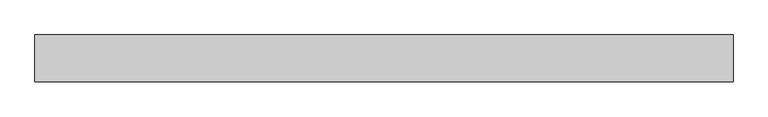
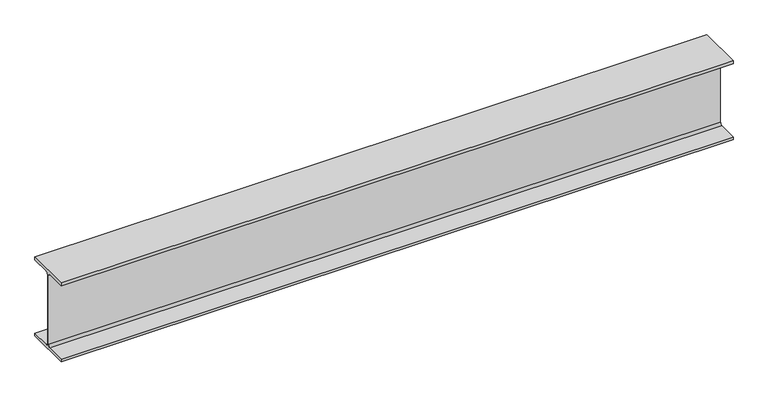
"""IFC4 building model written with IfcOpenShell, lengths in millimetres: beam geometry, Old_Steel Beam_H-KSD3502 : H_SB_ASB_H-194×150x6x9."""

import ifcopenshell
import ifcopenshell.guid

model = None  # the IFC model being written
_history = None  # IfcOwnerHistory: only IFC2X3 demands one
_inside = {}  # id of a spatial element -> (the spatial element, [elements in it])
_under = {}  # id of a project, library or spatial element -> (it, [spatial elements below it])
_declared = {}  # id of a project -> (the project, [libraries it declares])
_typed = {}  # id of a type object -> (the type object, [elements of that type])
_made_of = {}  # id of a material, layer set ... -> (it, [elements and type objects made of it])


def new_model(schema):
    """Start an empty IFC model of exactly this schema.

    Asked for "IFC4X3", IfcOpenShell would pick the latest addendum, in which some entities
    have other attributes; the version numbers below select the first issue.
    IFC2X3 requires an IfcOwnerHistory on every rooted entity: one is made here for all.
    """
    global model, _history
    if schema == "IFC4X3":
        model = ifcopenshell.file(schema_version=(4, 3, 0, 0))
    else:
        model = ifcopenshell.file(schema=schema)
    _inside.clear()
    _under.clear()
    _declared.clear()
    _typed.clear()
    _made_of.clear()
    _history = None
    if model.schema == "IFC2X3":
        org = make("IfcOrganization", Name="unknown")
        user = make(
            "IfcPersonAndOrganization",
            ThePerson=make("IfcPerson", FamilyName="unknown"),
            TheOrganization=org,
        )
        app = make(
            "IfcApplication",
            ApplicationDeveloper=org,
            Version="unknown",
            ApplicationFullName="unknown",
            ApplicationIdentifier="unknown",
        )
        _history = make(
            "IfcOwnerHistory",
            OwningUser=user,
            OwningApplication=app,
            ChangeAction="ADDED",
            CreationDate=0,
        )
    return model


def make(cls, **values):
    """One entity of the class cls with the attributes given. An attribute that is None is left unset."""
    return model.create_entity(
        cls, **{name: value for name, value in values.items() if value is not None}
    )


def rooted(cls, **values):
    """An entity with a GlobalId (a new one), such as an element, a storey or a relation."""
    return make(cls, GlobalId=ifcopenshell.guid.new(), OwnerHistory=_history, **values)


def si_unit(unit_type, name, prefix=None):
    """IfcSIUnit, for example si_unit("LENGTHUNIT", "METRE", prefix="MILLI")."""
    return make("IfcSIUnit", UnitType=unit_type, Prefix=prefix, Name=name)


def assignment(units):
    """IfcUnitAssignment: the units of a project."""
    return None if units is None else make("IfcUnitAssignment", Units=units)


def point(xyz):
    """IfcCartesianPoint."""
    return None if xyz is None else make("IfcCartesianPoint", Coordinates=xyz)


def direction(xyz):
    """IfcDirection."""
    return None if xyz is None else make("IfcDirection", DirectionRatios=xyz)


def frame(location, z_axis=None, x_axis=None):
    """IfcAxis2Placement3D, a coordinate frame: its origin and axes. An axis left out is left unset."""
    return make(
        "IfcAxis2Placement3D",
        Location=point(location),
        Axis=direction(z_axis),
        RefDirection=direction(x_axis),
    )


def frame_2d(location, x_axis=None):
    """IfcAxis2Placement2D, a coordinate frame in the plane: its origin and x axis."""
    return make(
        "IfcAxis2Placement2D", Location=point(location), RefDirection=direction(x_axis)
    )


def origin():
    """The frame at (0, 0, 0) with its axes left unset."""
    return frame((0.0, 0.0, 0.0))


def place(relative_to, where):
    """IfcLocalPlacement: puts the frame where relative to a parent placement (None: the world)."""
    return make(
        "IfcLocalPlacement", PlacementRelTo=relative_to, RelativePlacement=where
    )


def context(
    kind, dimensions, precision=None, world=None, true_north=None, identifier=None
):
    """IfcGeometricRepresentationContext, for example the 3D "Model" context."""
    return make(
        "IfcGeometricRepresentationContext",
        ContextIdentifier=identifier,
        ContextType=kind,
        CoordinateSpaceDimension=dimensions,
        Precision=precision,
        WorldCoordinateSystem=world,
        TrueNorth=true_north,
    )


def project(units=None, contexts=None):
    """IfcProject with its units and contexts."""
    return rooted(
        "IfcProject",
        Name="project",
        RepresentationContexts=contexts,
        UnitsInContext=assignment(units),
    )


def spatial(cls, under=None, at=None, **own):
    """A site, building, storey or space (cls), placed at a placement, below another one or the project."""
    s = rooted(cls, ObjectPlacement=at, **own)
    if under is not None:
        _under.setdefault(under.id(), (under, []))[1].append(s)
    return s


def polyline(points):
    """IfcPolyline through the points."""
    return make("IfcPolyline", Points=[point(p) for p in points])


def circle_curve(where, radius):
    """IfcCircle in the frame where."""
    return make("IfcCircle", Position=where, Radius=radius)


def trimmed(basis, trim1, trim2, sense, master):
    """IfcTrimmedCurve: the piece of a basis curve between two trims."""
    return make(
        "IfcTrimmedCurve",
        BasisCurve=basis,
        Trim1=trim1,
        Trim2=trim2,
        SenseAgreement=sense,
        MasterRepresentation=master,
    )


def segment(curve, same_sense, transition):
    """IfcCompositeCurveSegment."""
    return make(
        "IfcCompositeCurveSegment",
        Transition=transition,
        SameSense=same_sense,
        ParentCurve=curve,
    )


def composite_curve(segments, self_intersect=None):
    """IfcCompositeCurve: segments joined end to end."""
    return make("IfcCompositeCurve", Segments=segments, SelfIntersect=self_intersect)


def outline(outer, holes=None, kind="AREA"):
    """IfcArbitraryClosedProfileDef: a profile drawn as a closed curve; with holes, ...WithVoids."""
    if holes is None:
        return make("IfcArbitraryClosedProfileDef", ProfileType=kind, OuterCurve=outer)
    return make(
        "IfcArbitraryProfileDefWithVoids",
        ProfileType=kind,
        OuterCurve=outer,
        InnerCurves=holes,
    )


def extrude(swept, where, along, depth):
    """IfcExtrudedAreaSolid: the profile swept, set in the frame where, extruded along a direction by depth."""
    return make(
        "IfcExtrudedAreaSolid",
        SweptArea=swept,
        Position=where,
        ExtrudedDirection=direction(along),
        Depth=depth,
    )


def shape(context_of_items, identifier, shape_type, items):
    """IfcShapeRepresentation: the items that make up one representation, for example the "Body"."""
    return make(
        "IfcShapeRepresentation",
        ContextOfItems=context_of_items,
        RepresentationIdentifier=identifier,
        RepresentationType=shape_type,
        Items=items,
    )


def source(mapping_origin, context_of_items, identifier, shape_type, items):
    """IfcRepresentationMap: a shape defined once, which mapped items show again and again."""
    return make(
        "IfcRepresentationMap",
        MappingOrigin=mapping_origin,
        MappedRepresentation=shape(context_of_items, identifier, shape_type, items),
    )


def transform(
    local_origin,
    x_axis=None,
    y_axis=None,
    z_axis=None,
    scale=None,
    scale2=None,
    scale3=None,
    uniform=True,
):
    """IfcCartesianTransformationOperator3D, or its non-uniform kind. x_axis, y_axis, z_axis: its Axis1, 2, 3."""
    if uniform:
        return make(
            "IfcCartesianTransformationOperator3D",
            Axis1=direction(x_axis),
            Axis2=direction(y_axis),
            LocalOrigin=point(local_origin),
            Scale=scale,
            Axis3=direction(z_axis),
        )
    return make(
        "IfcCartesianTransformationOperator3DnonUniform",
        Axis1=direction(x_axis),
        Axis2=direction(y_axis),
        LocalOrigin=point(local_origin),
        Scale=scale,
        Axis3=direction(z_axis),
        Scale2=scale2,
        Scale3=scale3,
    )


def mapped(mapping_source, mapping_target):
    """IfcMappedItem: shows the shape of a source again, moved by a transform."""
    return make(
        "IfcMappedItem", MappingSource=mapping_source, MappingTarget=mapping_target
    )


def made_of(thing, what):
    """Note that an element or type object is made of a material, layer set ...; save() writes the relation."""
    if what is not None:
        _made_of.setdefault(what.id(), (what, []))[1].append(thing)
    return thing


def element(
    cls,
    number,
    at=None,
    inside=None,
    cuts=None,
    type_object=None,
    material=None,
    context=None,
    identifier="Body",
    shape_type=None,
    held_by="IfcProductDefinitionShape",
    body=None,
    shapes=None,
    **own,
):
    """One element of the class cls, such as IfcWall. Its Tag is "e" and its number.

    at: its placement. inside: the storey or other place that contains it. cuts: it is an
    opening in that element (IfcRelVoidsElement). A single representation is given by context,
    identifier, shape_type and body (its items); several are given by shapes. held_by: the class
    of the entity that holds the representations. save() writes the other relations.
    """
    e = rooted(cls, Tag="e%d" % number, ObjectPlacement=at, **own)
    if body is not None:
        shapes = [shape(context, identifier, shape_type, body)]
    if shapes is not None:
        e.Representation = make(held_by, Representations=shapes)
    if inside is not None:
        _inside.setdefault(inside.id(), (inside, []))[1].append(e)
    if cuts is not None:
        rooted(
            "IfcRelVoidsElement", RelatingBuildingElement=cuts, RelatedOpeningElement=e
        )
    if type_object is not None:
        _typed.setdefault(type_object.id(), (type_object, []))[1].append(e)
    return made_of(e, material)


def aggregate(whole, parts):
    """IfcRelAggregates: a whole, such as a stair, and the parts it consists of."""
    return rooted("IfcRelAggregates", RelatingObject=whole, RelatedObjects=parts)


def save(model, path):
    """Write the relations noted so far, then the file.

    IfcRelAggregates (storeys below a building ...), IfcRelContainedInSpatialStructure (elements
    in a storey), IfcRelDefinesByType, IfcRelAssociatesMaterial and IfcRelDeclares: one each for
    every whole, place, type object, material and project.
    """
    for whole, parts in _under.values():
        aggregate(whole, parts)
    for where, things in _inside.values():
        rooted(
            "IfcRelContainedInSpatialStructure",
            RelatedElements=things,
            RelatingStructure=where,
        )
    for kind, things in _typed.values():
        rooted("IfcRelDefinesByType", RelatedObjects=things, RelatingType=kind)
    for what, things in _made_of.values():
        rooted("IfcRelAssociatesMaterial", RelatedObjects=things, RelatingMaterial=what)
    for by, libraries in _declared.values():
        rooted("IfcRelDeclares", RelatingContext=by, RelatedDefinitions=libraries)
    model.write(path)


def beam_56381f75(model_context):
    return source(origin(), model_context, "Body", "SweptSolid", [
        extrude(outline(composite_curve([segment(polyline([(82.5, -141.5), (82.5, -151.7), (-82.5, -151.7), (-82.5, -141.5), (-11.9, -141.5)]), True, "CONTINUOUS"), segment(trimmed(circle_curve(frame_2d((-11.9, -132.6)), 8.9), [point((-11.9, -141.5))], [point((-3.0, -132.6))], True, "CARTESIAN"), True, "CONTINUOUS"), segment(polyline([(-3.0, -132.6), (-3.0, 132.6)]), True, "CONTINUOUS"), segment(trimmed(circle_curve(frame_2d((-11.9, 132.6)), 8.9), [point((-3.0, 132.6))], [point((-11.9, 141.5))], True, "CARTESIAN"), True, "CONTINUOUS"), segment(polyline([(-11.9, 141.5), (-82.5, 141.5), (-82.5, 151.7), (82.5, 151.7), (82.5, 141.5), (11.9, 141.5)]), True, "CONTINUOUS"), segment(trimmed(circle_curve(frame_2d((11.9, 132.6)), 8.9), [point((11.9, 141.5))], [point((3.0, 132.6))], True, "CARTESIAN"), True, "CONTINUOUS"), segment(polyline([(3.0, 132.6), (3.0, -132.6)]), True, "CONTINUOUS"), segment(trimmed(circle_curve(frame_2d((11.9, -132.6)), 8.9), [point((3.0, -132.6))], [point((11.9, -141.5))], True, "CARTESIAN"), True, "CONTINUOUS"), segment(polyline([(11.9, -141.5), (82.5, -141.5)]), True, "CONTINUOUS")], self_intersect=False)), frame((-1200.0, 0.0, 0.0), z_axis=(1.0, 0.0, 0.0), x_axis=(0.0, 1.0, 0.0)), (0.0, 0.0, 1.0), 2448.0465428),
    ])


if __name__ == "__main__":
    model = new_model("IFC4")
    model_context = context("Model", 3, world=origin())
    ifc_project = project(units=[si_unit("LENGTHUNIT", "METRE", prefix="MILLI")], contexts=[model_context])
    site = spatial("IfcSite", under=ifc_project)
    building = spatial("IfcBuilding", under=site)
    placement = place(None, origin())
    beam_shape = beam_56381f75(model_context)
    element("IfcBeam", 1, ObjectType="Old_Steel Beam_H-KSD3502 : H_SB_ASB_H-194×150x6x9", at=placement, inside=building, context=model_context, shape_type="MappedRepresentation", body=[
        mapped(beam_shape, transform((0.0, 0.0, 0.0), x_axis=(1.0, 0.0, 0.0), y_axis=(0.0, 1.0, 0.0), z_axis=(0.0, 0.0, 1.0))),
    ])
    save(model, "model.ifc")

# Revit data of these elements
# Type "Old_Steel Beam_H-KSD3502 : H_SB_ASB_H-194×150x6x9"
#   Width = 15.0 cm
#   Web Thickness = 0.6 cm
#   Web Fillet = 1.3 cm
#   Warping Constant = 43316.0 cm⁶
#   Torsional Moment of Inertia = 8.622 cm⁴
#   Torsional Modulus = 1.0 cm³
#   Section Area = 39.01 cm²
#   Plastic Modulus weak axis = 104.0 cm³
#   Plastic Modulus strong axis = 309.0 cm³
#   Perimeter = 0.95 m²/m
#   Nominal Weight = 30.60 kgf/m
#   Moment of Inertia weak axis = 507.00 cm⁴
#   Moment of Inertia strong axis = 2690.00 cm⁴
#   Height = 19.4 cm
#   Flange Thickness = 0.9 cm
#   Elastic Modulus weak axis = 67.6 cm³
#   Elastic Modulus strong axis = 277.0 cm³
#   Centroid Vertical = 9.7 cm
#   Centroid Horizontal = 7.5 cm
#   Length [instance default] = 1.5240 m
#   Structural Material [instance default] = Steel, 45-345
#   Assembly Code = ""
# Element 1 (IfcBeam, "Old_Steel Beam_H-KSD3502 : H_SB_ASB_H-194×150x6x9")
#   Structural Material = none
# Materials
#   "Steel, 45-345": class "Metal", colour RGB 189 187 185, transparency 0, Description = "Steel 345 MPa", Cost = 0
